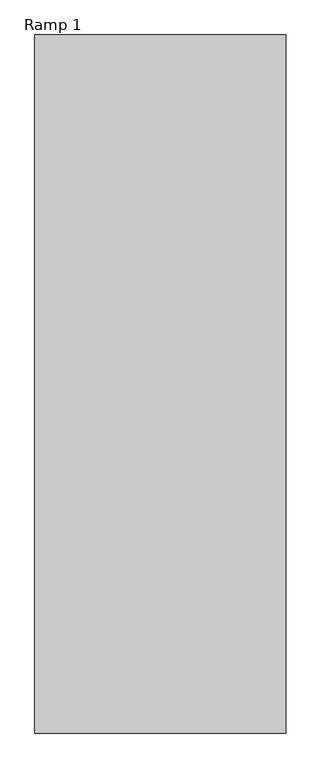
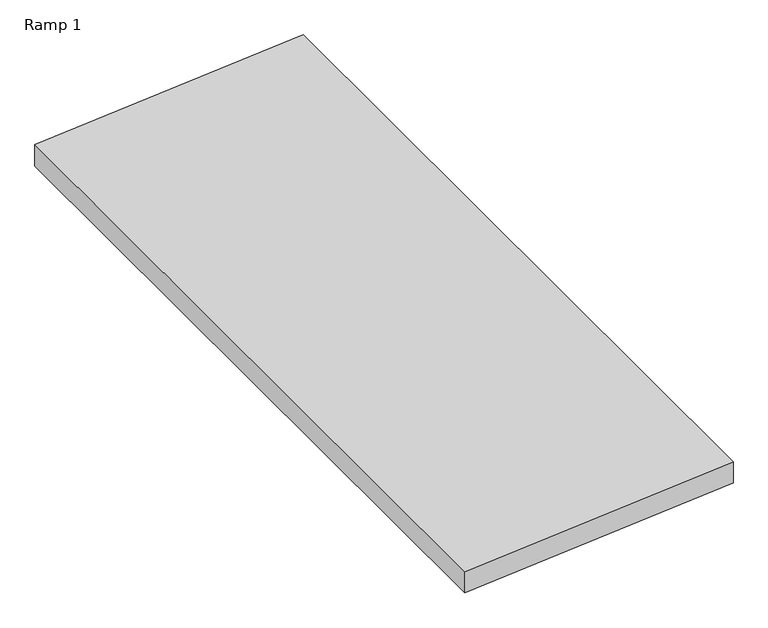
"""IFC4 building model written with IfcOpenShell, lengths in millimetres: ramp geometry, Ramp 1."""

from ifc_helpers import new_model, si_unit, frame, origin, place, context, project, spatial, polyline, outline, extrude, source, transform, mapped, element, save


def ramp_1_021fb7ed(model_context):
    return source(origin(), model_context, "Body", "SweptSolid", [
        extrude(outline(polyline([(150.0, -375.3), (0.0, -2175.3), (-150.5199322, -2175.3), (-0.5199322, -375.3), (150.0, -375.3)])), frame((0.0, 16577.264479, 0.0), z_axis=(0.0, 1.0, 0.0), x_axis=(0.0, 0.0, 1.0)), (0.0, 0.0, 1.0), 5000.0),
    ])


if __name__ == "__main__":
    model = new_model("IFC4")
    model_context = context("Model", 3, world=origin())
    ifc_project = project(units=[si_unit("LENGTHUNIT", "METRE", prefix="MILLI")], contexts=[model_context])
    site = spatial("IfcSite", under=ifc_project)
    building = spatial("IfcBuilding", under=site)
    placement = place(None, origin())
    ramp_1_shape = ramp_1_021fb7ed(model_context)
    element("IfcRamp", 1, ObjectType="Ramp 1", at=placement, inside=building, context=model_context, shape_type="MappedRepresentation", body=[
        mapped(ramp_1_shape, transform((0.0, 0.0, 0.0), x_axis=(1.0, 0.0, 0.0), y_axis=(0.0, 1.0, 0.0), z_axis=(0.0, 0.0, 1.0))),
    ])
    save(model, "model.ifc")
